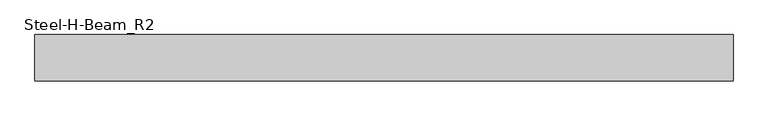
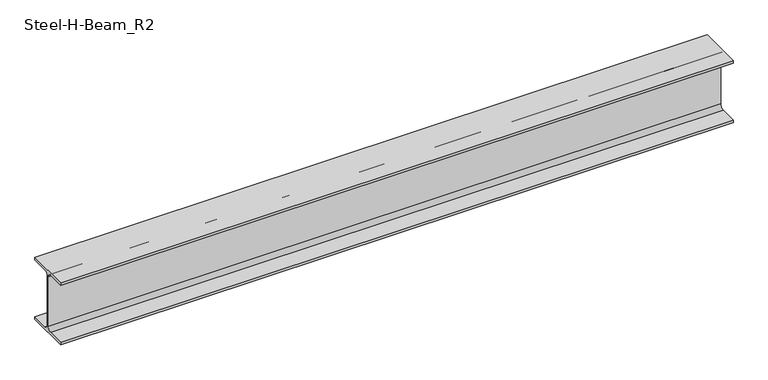
"""IFC4 building model written with IfcOpenShell, lengths in millimetres: beam geometry, Steel-H-Beam_R2 : BM121_H-294×200x8x12_SB1."""

from ifc_helpers import new_model, si_unit, point, frame, frame_2d, origin, place, context, project, spatial, polyline, circle_curve, trimmed, segment, composite_curve, outline, extrude, source, transform, mapped, element, save


def steel_h_beam_r2_827bf599(model_context):
    return source(origin(), model_context, "Body", "SweptSolid", [
        extrude(outline(composite_curve([segment(polyline([(100.0, -135.0), (100.0, -147.0), (-100.0, -147.0), (-100.0, -135.0), (-22.0, -135.0)]), True, "CONTINUOUS"), segment(trimmed(circle_curve(frame_2d((-22.0, -117.0)), 18.0), [point((-22.0, -135.0))], [point((-4.0, -117.0))], True, "CARTESIAN"), True, "CONTINUOUS"), segment(polyline([(-4.0, -117.0), (-4.0, 117.0)]), True, "CONTINUOUS"), segment(trimmed(circle_curve(frame_2d((-22.0, 117.0)), 18.0), [point((-4.0, 117.0))], [point((-22.0, 135.0))], True, "CARTESIAN"), True, "CONTINUOUS"), segment(polyline([(-22.0, 135.0), (-100.0, 135.0), (-100.0, 147.0), (100.0, 147.0), (100.0, 135.0), (22.0, 135.0)]), True, "CONTINUOUS"), segment(trimmed(circle_curve(frame_2d((22.0, 117.0)), 18.0), [point((22.0, 135.0))], [point((4.0, 117.0))], True, "CARTESIAN"), True, "CONTINUOUS"), segment(polyline([(4.0, 117.0), (4.0, -117.0)]), True, "CONTINUOUS"), segment(trimmed(circle_curve(frame_2d((22.0, -117.0)), 18.0), [point((4.0, -117.0))], [point((22.0, -135.0))], True, "CARTESIAN"), True, "CONTINUOUS"), segment(polyline([(22.0, -135.0), (100.0, -135.0)]), True, "CONTINUOUS")], self_intersect=False)), frame((-1512.3, 0.0, 0.0), z_axis=(1.0, 0.0, 0.0), x_axis=(0.0, 1.0, 0.0)), (0.0, 0.0, 1.0), 3012.3),
    ])


if __name__ == "__main__":
    model = new_model("IFC4")
    model_context = context("Model", 3, world=origin())
    ifc_project = project(units=[si_unit("LENGTHUNIT", "METRE", prefix="MILLI")], contexts=[model_context])
    site = spatial("IfcSite", under=ifc_project)
    building = spatial("IfcBuilding", under=site)
    placement = place(None, origin())
    steel_h_beam_r2_shape = steel_h_beam_r2_827bf599(model_context)
    element("IfcBeam", 1, ObjectType="Steel-H-Beam_R2 : BM121_H-294×200x8x12_SB1", at=placement, inside=building, context=model_context, shape_type="MappedRepresentation", body=[
        mapped(steel_h_beam_r2_shape, transform((0.0, 0.0, 0.0), x_axis=(1.0, 0.0, 0.0), y_axis=(0.0, 1.0, 0.0), z_axis=(0.0, 0.0, 1.0))),
    ])
    save(model, "model.ifc")

# Revit data of these elements
# Type "Steel-H-Beam_R2 : BM121_H-294×200x8x12_SB1"
#   SteelWeight = "Medium"
#   Surface Area = 1.3411 m²/m
#   Section Area = 72.3812 cm²
#   Mass per Unit Length = 56.8193 kg/m
#   Length [instance default] = 3000 mm
#   B = 200 mm
#   H = 294 mm
#   r = 18 mm
#   tw = 8 mm
#   tf = 12 mm
#   hec_material4 [instance default] = none
#   hec_material3 [instance default] = none
#   hec_material2 [instance default] = none
#   hec_material1 [instance default] = none
#   Structural Material [instance default] = Steel, 45-345
#   Assembly Code = ""
# Element 1 (IfcBeam, "Steel-H-Beam_R2 : BM121_H-294×200x8x12_SB1")
#   Materials on its faces: "Steel, 45-345"
# Materials
#   "Steel, 45-345": class "Metal", colour RGB 189 187 185, transparency 0, Description = "Steel 345 MPa", Cost = 0
